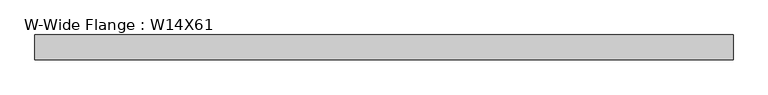
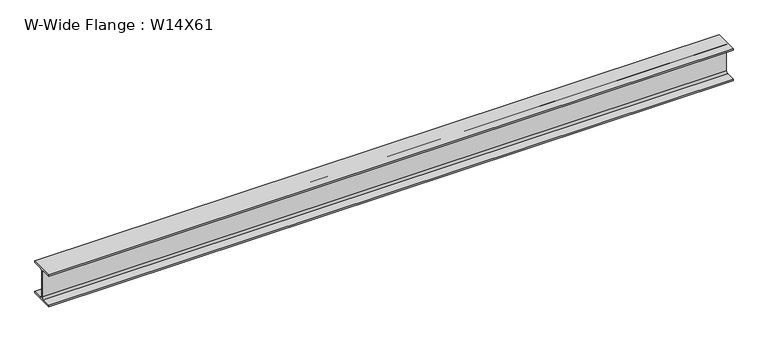
"""IFC4 building model written with IfcOpenShell, lengths in millimetres: beam geometry, W-Wide Flange : W14X61."""

from ifc_helpers import new_model, si_unit, point, frame, frame_2d, origin, place, context, project, spatial, polyline, circle_curve, trimmed, segment, composite_curve, outline, extrude, source, transform, mapped, element, save


def w_wide_flange_w14x61_86819d2a(model_context):
    return source(origin(), model_context, "Body", "SweptSolid", [
        extrude(outline(composite_curve([segment(polyline([(127.0, -160.147), (127.0, -176.53), (-127.0, -176.53), (-127.0, -160.147), (-26.4795, -160.147)]), True, "CONTINUOUS"), segment(trimmed(circle_curve(frame_2d((-26.4795, -138.43)), 21.717), [point((-26.4795, -160.147))], [point((-4.7625, -138.43))], True, "CARTESIAN"), True, "CONTINUOUS"), segment(polyline([(-4.7625, -138.43), (-4.7625, 138.43)]), True, "CONTINUOUS"), segment(trimmed(circle_curve(frame_2d((-26.4795, 138.43)), 21.717), [point((-4.7625, 138.43))], [point((-26.4795, 160.147))], True, "CARTESIAN"), True, "CONTINUOUS"), segment(polyline([(-26.4795, 160.147), (-127.0, 160.147), (-127.0, 176.53), (127.0, 176.53), (127.0, 160.147), (26.4795, 160.147)]), True, "CONTINUOUS"), segment(trimmed(circle_curve(frame_2d((26.4795, 138.43)), 21.717), [point((26.4795, 160.147))], [point((4.7625, 138.43))], True, "CARTESIAN"), True, "CONTINUOUS"), segment(polyline([(4.7625, 138.43), (4.7625, -138.43)]), True, "CONTINUOUS"), segment(trimmed(circle_curve(frame_2d((26.4795, -138.43)), 21.717), [point((4.7625, -138.43))], [point((26.4795, -160.147))], True, "CARTESIAN"), True, "CONTINUOUS"), segment(polyline([(26.4795, -160.147), (127.0, -160.147)]), True, "CONTINUOUS")], self_intersect=False)), frame((-3510.7066406, 0.0, 0.0), z_axis=(1.0, 0.0, 0.0), x_axis=(0.0, 1.0, 0.0)), (0.0, 0.0, 1.0), 7156.3507813),
    ])


if __name__ == "__main__":
    model = new_model("IFC4")
    model_context = context("Model", 3, world=origin())
    ifc_project = project(units=[si_unit("LENGTHUNIT", "METRE", prefix="MILLI")], contexts=[model_context])
    site = spatial("IfcSite", under=ifc_project)
    building = spatial("IfcBuilding", under=site)
    placement = place(None, origin())
    w_wide_flange_w14x61_shape = w_wide_flange_w14x61_86819d2a(model_context)
    element("IfcBeam", 1, ObjectType="W-Wide Flange : W14X61", at=placement, inside=building, context=model_context, shape_type="MappedRepresentation", body=[
        mapped(w_wide_flange_w14x61_shape, transform((0.0, 0.0, 0.0), x_axis=(1.0, 0.0, 0.0), y_axis=(0.0, 1.0, 0.0), z_axis=(0.0, 0.0, 1.0))),
    ])
    save(model, "model.ifc")

# Revit data of these elements
# Type "W-Wide Flange : W14X61"
#   Assembly Code = "B10"
#   W = 61
#   Length [instance default] = 1524 mm
#   bf = 254 mm
#   d = 353.06 mm
#   k = 38.1 mm
#   k2 = 21.717 mm
#   tf = 16.383 mm
#   tw = 9.525 mm
#   A = 0.0115484 m²
#   Structural Material [instance default] = Steel ASTM A992
# Element 1 (IfcBeam, "W-Wide Flange : W14X61")
#   Structural Material = Aluminum, Anodized Red
#   Materials on its faces: "Aluminum, Anodized Red"
# Materials
#   "Steel ASTM A992": class "Metal", colour RGB 128 0 0, transparency 0, Description = "Structural steel 50ksi", Cost = 0
#   "Aluminum, Anodized Red": class "Metal", colour RGB 120 120 120, transparency 0, Description = "Anodized aluminum, red", Cost = 0
